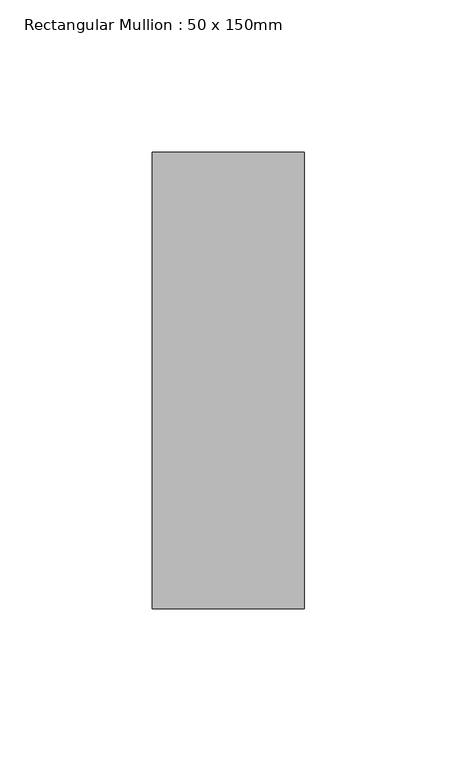
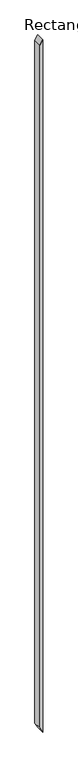
"""IFC4 building model written with IfcOpenShell, lengths in millimetres: member geometry, Rectangular Mullion : 50 x 150mm."""

from ifc_helpers import new_model, si_unit, frame, origin, place, context, project, spatial, polyline, outline, extrude, source, transform, mapped, element, save


def rectangular_mullion_50_x_150mm_06c78d0c(model_context):
    return source(origin(), model_context, "Body", "SweptSolid", [
        extrude(outline(polyline([(0.0, 0.0), (-83.6497392, -50.0), (-12851.6468426, -50.0), (-12948.4045305, 0.0), (0.0, 0.0)])), frame((0.0, -75.0, 0.0), z_axis=(0.0, 1.0, 0.0), x_axis=(0.0, 0.0, 1.0)), (0.0, 0.0, 1.0), 150.0),
    ])


if __name__ == "__main__":
    model = new_model("IFC4")
    model_context = context("Model", 3, world=origin())
    ifc_project = project(units=[si_unit("LENGTHUNIT", "METRE", prefix="MILLI")], contexts=[model_context])
    site = spatial("IfcSite", under=ifc_project)
    building = spatial("IfcBuilding", under=site)
    placement = place(None, origin())
    rectangular_mullion_50_x_150mm_shape = rectangular_mullion_50_x_150mm_06c78d0c(model_context)
    element("IfcMember", 1, ObjectType="Rectangular Mullion : 50 x 150mm", at=placement, inside=building, context=model_context, shape_type="MappedRepresentation", body=[
        mapped(rectangular_mullion_50_x_150mm_shape, transform((0.0, 0.0, 0.0), x_axis=(1.0, 0.0, 0.0), y_axis=(0.0, 1.0, 0.0), z_axis=(0.0, 0.0, 1.0))),
    ])
    save(model, "model.ifc")

# Revit data of these elements
# Type "Rectangular Mullion : 50 x 150mm"
#   built-in parameter 1007304 = 0.492126 (stored number, unit not read)
#   built-in parameter 1007301 = 0.082021 (stored number, unit not read)
#   built-in parameter 1007300 = 0.082021 (stored number, unit not read)
# Element 1 (IfcMember, "Rectangular Mullion : 50 x 150mm")
#   Materials on its faces: "Metal - Aluminium"
# Materials
#   "Metal - Aluminium": class "Metal", colour RGB 247 247 247, transparency 0
